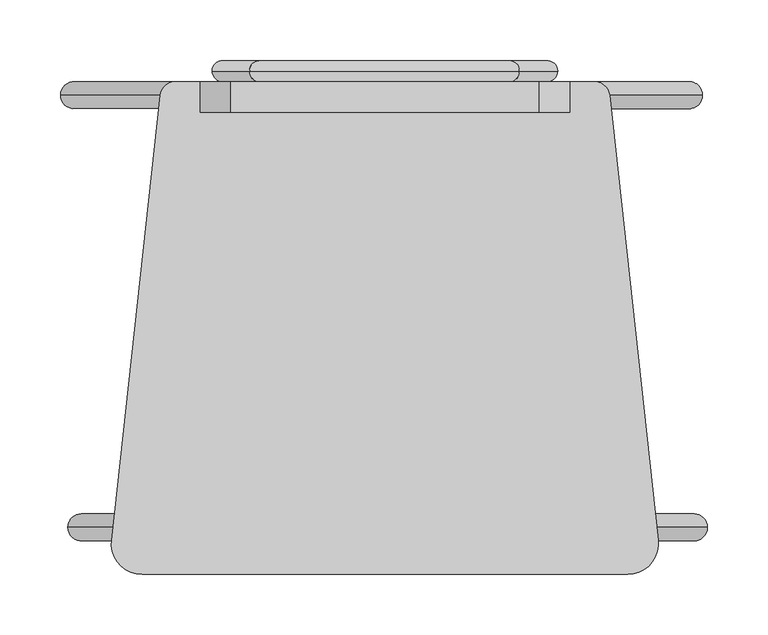
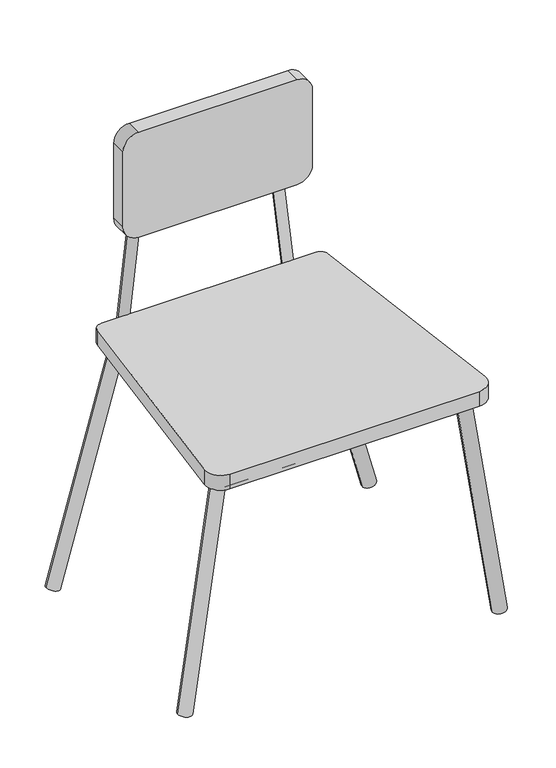
"""IFC4 building model written with IfcOpenShell, lengths in millimetres: furniture geometry, Stuhl - Schüler - Mittel : Stuhl - Schüler - Mittel."""

from ifc_helpers import new_model, si_unit, point, frame, frame_2d, origin, place, context, project, spatial, polyline, circle_curve, ellipse_curve, trimmed, segment, composite_curve, outline, extrude, source, transform, mapped, element, save
from ifc_brep_helpers import plane_surface, cylinder_surface, advanced_brep


def furniture_cd35c0ec(model_context):
    return source(origin(), model_context, "Body", "SolidModel", [
        advanced_brep(
        [(-246.1119338, 141.3112884, -2.9762313), (-267.5249862, 141.3112884, 2.9762313), (-143.9552174, 141.3112884, 364.5165709), (-160.8447826, 141.3112884, 386.7415709), (143.8319962, 141.3112884, 364.5165709), (160.9680038, 141.3112884, 386.7415709), (240.434444, 141.3112884, -2.8262314), (261.928636, 141.3112884, 2.8262314)],
        [
            (0, 1, circle_curve(frame((-256.81846, 141.3112884, 0.0), z_axis=(-0.2678273342991428, 0.0, -0.9634669267817215), x_axis=(-0.9634669267817215, 0.0, 0.2678273342991428)), 11.1125)),
            (1, 0, circle_curve(frame((-256.81846, 141.3112884, 0.0), z_axis=(-0.2678273342991428, 0.0, -0.9634669267817215), x_axis=(-0.9634669267817215, 0.0, 0.2678273342991428)), 11.1125)),
            (0, 2),
            (2, 3, ellipse_curve(frame((-152.4, 141.3112884, 375.6290709), z_axis=(-0.7961869548978878, 0.0, -0.6050506861829252), x_axis=(0.6050506861829252, 0.0, -0.796186954897888)), 13.957149, 11.1125)),
            (3, 1),
            (3, 2, ellipse_curve(frame((-152.4, 141.3112884, 375.6290709), z_axis=(-0.7961869548978878, 0.0, -0.6050506861829252), x_axis=(0.6050506861829252, 0.0, -0.796186954897888)), 13.957149, 11.1125)),
            (2, 4),
            (4, 5, ellipse_curve(frame((152.4, 141.3112884, 375.6290709), z_axis=(-0.7919371941469172, 0.0, 0.610602555290025), x_axis=(-0.6106025552900248, 0.0, -0.7919371941469173)), 14.0320471, 11.1125)),
            (5, 3),
            (5, 4, ellipse_curve(frame((152.4, 141.3112884, 375.6290709), z_axis=(-0.7919371941469172, 0.0, 0.610602555290025), x_axis=(-0.6106025552900248, 0.0, -0.7919371941469173)), 14.0320471, 11.1125)),
            (6, 7, circle_curve(frame((251.18154, 141.3112884, 0.0), z_axis=(0.2543290389465838, 0.0, -0.9671177487506406), x_axis=(0.9671177487506406, 0.0, 0.2543290389465838)), 11.1125)),
            (7, 6, circle_curve(frame((251.18154, 141.3112884, 0.0), z_axis=(0.2543290389465838, 0.0, -0.9671177487506406), x_axis=(0.9671177487506406, 0.0, 0.2543290389465838)), 11.1125)),
            (4, 6),
            (7, 5),
        ],
        [
            plane_surface(frame((-256.81846, 104.4181887, 0.0), z_axis=(-0.26782733429914296, 0.0, -0.9634669267817215), x_axis=(0.9634669267817215, 0.0, -0.26782733429914296))),
            cylinder_surface(frame((-256.81846, 141.3112884, 0.0), z_axis=(-0.2678273342991428, 0.0, -0.9634669267817215), x_axis=(-0.9634669267817215, 0.0, 0.2678273342991428)), 11.1125),
            cylinder_surface(frame((-152.4, 141.3112884, 375.6290709), z_axis=(-1.0, 0.0, 0.0), x_axis=(0.0, 0.0, 1.0)), 11.1125),
            plane_surface(frame((251.18154, 151.5986679, 0.0), z_axis=(0.25432903894658365, 0.0, -0.9671177487506406), x_axis=(0.9671177487506406, 0.0, 0.25432903894658365))),
            cylinder_surface(frame((152.4, 141.3112884, 375.6290709), z_axis=(-0.2543290389465838, 0.0, 0.9671177487506406), x_axis=(0.9671177487506406, 0.0, 0.2543290389465838)), 11.1125),
        ],
        [
            (0, [[1, 2]]),
            (1, [[-1, 3, 4, 5]]),
            (1, [[-2, -5, 6, -3]]),
            (2, [[-4, 7, 8, 9]]),
            (2, [[-6, -9, 10, -7]]),
            (3, [[11, 12]]),
            (4, [[-8, 13, -12, 14]]),
            (4, [[-10, -14, -11, -13]]),
        ],
    ),
        extrude(outline(composite_curve([segment(trimmed(circle_curve(frame_2d((711.2, -127.0)), 25.4), [point((736.6, -127.0))], [point((711.2, -152.4))], False, "CARTESIAN"), True, "CONTINUOUS"), segment(polyline([(711.2, -152.4), (583.5915709, -152.4)]), True, "CONTINUOUS"), segment(trimmed(circle_curve(frame_2d((583.5915709, -127.0)), 25.4), [point((583.5915709, -152.4))], [point((558.1915709, -127.0))], False, "CARTESIAN"), True, "CONTINUOUS"), segment(polyline([(558.1915709, -127.0), (558.1915709, 127.0)]), True, "CONTINUOUS"), segment(trimmed(circle_curve(frame_2d((583.5915709, 127.0)), 25.4), [point((558.1915709, 127.0))], [point((583.5915709, 152.4))], False, "CARTESIAN"), True, "CONTINUOUS"), segment(polyline([(583.5915709, 152.4), (711.2, 152.4)]), True, "CONTINUOUS"), segment(trimmed(circle_curve(frame_2d((711.2, 127.0)), 25.4), [point((711.2, 152.4))], [point((736.6, 127.0))], False, "CARTESIAN"), True, "CONTINUOUS"), segment(polyline([(736.6, 127.0), (736.6, -127.0)]), True, "CONTINUOUS")], self_intersect=False)), frame((0.0, 127.0, 0.0), z_axis=(0.0, 1.0, 0.0), x_axis=(0.0, 0.0, 1.0)), (0.0, 0.0, 1.0), 25.4),
        advanced_brep(
        [(125.2918104, 161.0495808, 385.7808371), (142.4839294, 161.0495808, 387.7023047), (95.5658681, 161.0495808, 651.7504192), (111.0393076, 161.0495808, 669.0495808), (-96.1094419, 161.0495808, 651.7504192), (-111.614346, 161.0495808, 669.0495808), (-125.2898881, 161.0495808, 385.7981949), (-142.4858516, 161.0495808, 387.6849469)],
        [
            (0, 1, circle_curve(frame((133.8878699, 161.0495808, 386.7415709), z_axis=(0.11107287460648643, 0.0, -0.9938122642263235), x_axis=(0.9938122642263235, 0.0, 0.11107287460648643)), 8.6495808)),
            (1, 0, circle_curve(frame((133.8878699, 161.0495808, 386.7415709), z_axis=(0.11107287460648643, 0.0, -0.9938122642263235), x_axis=(0.9938122642263235, 0.0, 0.11107287460648643)), 8.6495808)),
            (0, 2),
            (2, 3, ellipse_curve(frame((103.3025878, 161.0495808, 660.4), z_axis=(0.7453431674760594, 0.0, -0.6666810052017043), x_axis=(-0.6666810052017043, 0.0, -0.7453431674760594)), 11.6048301, 8.6495808)),
            (3, 1),
            (3, 2, ellipse_curve(frame((103.3025878, 161.0495808, 660.4), z_axis=(0.7453431674760594, 0.0, -0.6666810052017043), x_axis=(-0.6666810052017043, 0.0, -0.7453431674760594)), 11.6048301, 8.6495808)),
            (2, 4),
            (4, 5, ellipse_curve(frame((-103.8618939, 161.0495808, 660.4), z_axis=(0.7446697570428843, 0.0, 0.6674331074689747), x_axis=(0.6674331074689746, 0.0, -0.7446697570428844)), 11.6153244, 8.6495808)),
            (5, 3),
            (5, 4, ellipse_curve(frame((-103.8618939, 161.0495808, 660.4), z_axis=(0.7446697570428843, 0.0, 0.6674331074689747), x_axis=(0.6674331074689746, 0.0, -0.7446697570428844)), 11.6153244, 8.6495808)),
            (6, 7, circle_curve(frame((-133.8878699, 161.0495808, 386.7415709), z_axis=(-0.10906609410862052, 0.0, -0.9940344999625966), x_axis=(-0.9940344999625966, 0.0, 0.10906609410862052)), 8.6495808)),
            (7, 6, circle_curve(frame((-133.8878699, 161.0495808, 386.7415709), z_axis=(-0.10906609410862052, 0.0, -0.9940344999625966), x_axis=(-0.9940344999625966, 0.0, 0.10906609410862052)), 8.6495808)),
            (4, 6),
            (7, 5),
        ],
        [
            plane_surface(frame((133.8878699, 135.690293, 386.7415709), z_axis=(0.11107287460648242, 0.0, -0.993812264226324), x_axis=(0.993812264226324, 0.0, 0.11107287460648242))),
            cylinder_surface(frame((133.8878699, 161.0495808, 386.7415709), z_axis=(0.11107287460648643, 0.0, -0.9938122642263235), x_axis=(0.9938122642263235, 0.0, 0.11107287460648643)), 8.6495808),
            cylinder_surface(frame((103.3025878, 161.0495808, 660.4), z_axis=(1.0, 0.0, 0.0), x_axis=(0.0, 0.0, 1.0)), 8.6495808),
            plane_surface(frame((-133.8878699, 169.109707, 386.7415709), z_axis=(-0.10906609410862456, 0.0, -0.9940344999625962), x_axis=(0.9940344999625962, 0.0, -0.10906609410862456))),
            cylinder_surface(frame((-103.8618939, 161.0495808, 660.4), z_axis=(0.10906609410862052, 0.0, 0.9940344999625966), x_axis=(-0.9940344999625966, 0.0, 0.10906609410862052)), 8.6495808),
        ],
        [
            (0, [[1, 2]]),
            (1, [[-1, 3, 4, 5]]),
            (1, [[-2, -5, 6, -3]]),
            (2, [[-4, 7, 8, 9]]),
            (2, [[-6, -9, 10, -7]]),
            (3, [[11, 12]]),
            (4, [[-8, 13, -12, 14]]),
            (4, [[-10, -14, -11, -13]]),
        ],
    ),
        advanced_brep(
        [(-239.4674707, -215.2971399, -1.5703154), (-261.4694493, -215.2971399, 1.5703154), (-187.2110918, -215.2971399, 364.5165709), (-206.4889082, -215.2971399, 386.7415709), (187.3282624, -215.2971399, 364.5165709), (206.3717376, -215.2971399, 386.7415709), (244.1320967, -215.2971399, -1.7032764), (266.0944741, -215.2971399, 1.7032764)],
        [
            (0, 1, circle_curve(frame((-250.46846, -215.2971399, 0.0), z_axis=(-0.14131071990492466, 0.0, -0.9899652925431033), x_axis=(-0.9899652925431033, 0.0, 0.14131071990492466)), 11.1125)),
            (1, 0, circle_curve(frame((-250.46846, -215.2971399, 0.0), z_axis=(-0.14131071990492466, 0.0, -0.9899652925431033), x_axis=(-0.9899652925431033, 0.0, 0.14131071990492466)), 11.1125)),
            (0, 2),
            (2, 3, ellipse_curve(frame((-196.85, -215.2971399, 375.6290709), z_axis=(-0.7554173415751471, 0.0, -0.6552439546058687), x_axis=(0.6552439546058687, 0.0, -0.7554173415751468)), 14.7104116, 11.1125)),
            (3, 1),
            (3, 2, ellipse_curve(frame((-196.85, -215.2971399, 375.6290709), z_axis=(-0.7554173415751471, 0.0, -0.6552439546058687), x_axis=(0.6552439546058687, 0.0, -0.7554173415751468)), 14.7104116, 11.1125)),
            (2, 4),
            (4, 5, ellipse_curve(frame((196.85, -215.2971399, 375.6290709), z_axis=(-0.759366748266108, 0.0, 0.6506628478926374), x_axis=(-0.6506628478926374, 0.0, -0.759366748266108)), 14.6339039, 11.1125)),
            (5, 3),
            (5, 4, ellipse_curve(frame((196.85, -215.2971399, 375.6290709), z_axis=(-0.759366748266108, 0.0, 0.6506628478926374), x_axis=(-0.6506628478926374, 0.0, -0.759366748266108)), 14.6339039, 11.1125)),
            (6, 7, circle_curve(frame((255.1132854, -215.2971399, 0.0), z_axis=(0.15327571674448523, 0.0, -0.9881834620435946), x_axis=(0.9881834620435946, 0.0, 0.15327571674448523)), 11.1125)),
            (7, 6, circle_curve(frame((255.1132854, -215.2971399, 0.0), z_axis=(0.15327571674448523, 0.0, -0.9881834620435946), x_axis=(0.9881834620435946, 0.0, 0.15327571674448523)), 11.1125)),
            (4, 6),
            (7, 5),
        ],
        [
            plane_surface(frame((-250.46846, -252.1902396, 0.0), z_axis=(-0.1413107199049246, 0.0, -0.9899652925431033), x_axis=(0.9899652925431033, 0.0, -0.1413107199049246))),
            cylinder_surface(frame((-250.46846, -215.2971399, 0.0), z_axis=(-0.14131071990492466, 0.0, -0.9899652925431033), x_axis=(-0.9899652925431033, 0.0, 0.14131071990492466)), 11.1125),
            cylinder_surface(frame((-196.85, -215.2971399, 375.6290709), z_axis=(-1.0, 0.0, 0.0), x_axis=(0.0, 0.0, 1.0)), 11.1125),
            plane_surface(frame((255.1132854, -205.0097604, 0.0), z_axis=(0.1532757167444853, 0.0, -0.9881834620435946), x_axis=(0.9881834620435946, 0.0, 0.1532757167444853))),
            cylinder_surface(frame((196.85, -215.2971399, 375.6290709), z_axis=(-0.15327571674448523, 0.0, 0.9881834620435946), x_axis=(0.9881834620435946, 0.0, 0.15327571674448523)), 11.1125),
        ],
        [
            (0, [[1, 2]]),
            (1, [[-1, 3, 4, 5]]),
            (1, [[-2, -5, 6, -3]]),
            (2, [[-4, 7, 8, 9]]),
            (2, [[-6, -9, 10, -7]]),
            (3, [[11, 12]]),
            (4, [[-8, 13, -12, 14]]),
            (4, [[-10, -14, -11, -13]]),
        ],
    ),
        extrude(outline(composite_curve([segment(trimmed(circle_curve(frame_2d((172.7689225, 139.7)), 12.7), [point((172.7689225, 152.4))], [point((185.3936523, 141.0806509))], False, "CARTESIAN"), True, "CONTINUOUS"), segment(polyline([(185.3936523, 141.0806509), (225.5202567, -225.8386982)]), True, "CONTINUOUS"), segment(trimmed(circle_curve(frame_2d((200.270797, -228.6)), 25.4), [point((225.5202567, -225.8386982))], [point((200.270797, -254.0))], False, "CARTESIAN"), True, "CONTINUOUS"), segment(polyline([(200.270797, -254.0), (-200.270797, -254.0)]), True, "CONTINUOUS"), segment(trimmed(circle_curve(frame_2d((-200.270797, -228.6)), 25.4), [point((-200.270797, -254.0))], [point((-225.5202567, -225.8386982))], False, "CARTESIAN"), True, "CONTINUOUS"), segment(polyline([(-225.5202567, -225.8386982), (-185.3936523, 141.0806509)]), True, "CONTINUOUS"), segment(trimmed(circle_curve(frame_2d((-172.7689225, 139.7)), 12.7), [point((-185.3936523, 141.0806509))], [point((-172.7689225, 152.4))], False, "CARTESIAN"), True, "CONTINUOUS"), segment(polyline([(-172.7689225, 152.4), (172.7689225, 152.4)]), True, "CONTINUOUS")], self_intersect=False)), frame((0.0, 0.0, 386.7415709), z_axis=(0.0, 0.0, 1.0), x_axis=(1.0, 0.0, 0.0)), (0.0, 0.0, 1.0), 25.4),
    ])


if __name__ == "__main__":
    model = new_model("IFC4")
    model_context = context("Model", 3, world=origin())
    ifc_project = project(units=[si_unit("LENGTHUNIT", "METRE", prefix="MILLI")], contexts=[model_context])
    site = spatial("IfcSite", under=ifc_project)
    building = spatial("IfcBuilding", under=site)
    placement = place(None, origin())
    furniture_shape = furniture_cd35c0ec(model_context)
    element("IfcFurniture", 1, ObjectType="Stuhl - Schüler - Mittel : Stuhl - Schüler - Mittel", at=placement, inside=building, context=model_context, shape_type="MappedRepresentation", body=[
        mapped(furniture_shape, transform((0.0, 0.0, 0.0), x_axis=(1.0, 0.0, 0.0), y_axis=(0.0, 1.0, 0.0), z_axis=(0.0, 0.0, 1.0))),
    ])
    save(model, "model.ifc")

# Revit data of these elements
# Type "Stuhl - Schüler - Mittel : Stuhl - Schüler - Mittel"
#   Material = Holz - Eiche
#   Assembly Code = ""
# Element 1 (IfcFurniture, "Stuhl - Schüler - Mittel : Stuhl - Schüler - Mittel")
#   Materials on its faces: "Metall - Chrom", "Holz - Eiche"
# Materials
#   "Holz - Eiche": class "Holz", colour RGB 128 64 0, transparency 0, Cost = 0
#   "Metall - Chrom": class "Metall", colour RGB 247 247 247, transparency 0, Cost = 0
